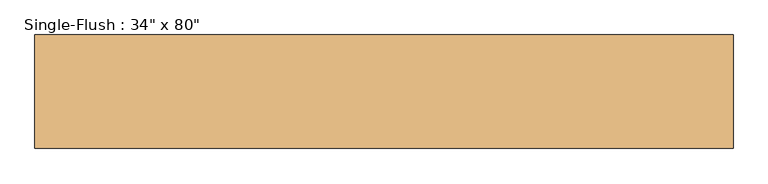
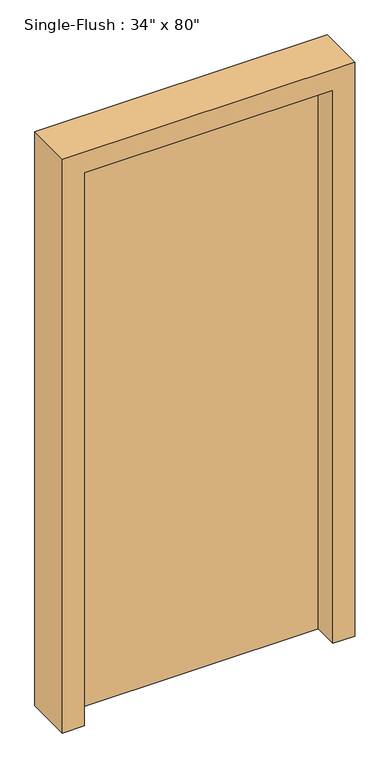
"""IFC4 building model written with IfcOpenShell, lengths in millimetres: door geometry."""

from ifc_helpers import new_model, si_unit, frame, origin, origin_with_axes, place, context, project, spatial, polyline, outline, extrude, source, transform, mapped, element, save


def door_d19e2db2(model_context):
    return source(origin(), model_context, "Body", "SweptSolid", [
        extrude(outline(polyline([(2108.2, 508.0), (2108.2, -508.0), (0.0, -508.0), (0.0, -431.8), (2032.0, -431.8), (2032.0, 431.8), (0.0, 431.8), (0.0, 508.0), (2108.2, 508.0)])), frame((0.0, -82.55, 0.0), z_axis=(0.0, 1.0, 0.0), x_axis=(0.0, 0.0, 1.0)), (0.0, 0.0, 1.0), 165.1),
        extrude(outline(polyline([(431.8, 6.35), (-431.8, 6.35), (-431.8, 57.15), (431.8, 57.15), (431.8, 6.35)])), origin_with_axes(), (0.0, 0.0, 1.0), 2032.0),
    ])


if __name__ == "__main__":
    model = new_model("IFC4")
    model_context = context("Model", 3, world=origin())
    ifc_project = project(units=[si_unit("LENGTHUNIT", "METRE", prefix="MILLI")], contexts=[model_context])
    site = spatial("IfcSite", under=ifc_project)
    building = spatial("IfcBuilding", under=site)
    placement = place(None, origin())
    door_shape = door_d19e2db2(model_context)
    element("IfcDoor", 1, ObjectType="Single-Flush : 34\" x 80\"", at=placement, inside=building, context=model_context, shape_type="MappedRepresentation", body=[
        mapped(door_shape, transform((0.0, 0.0, 0.0), x_axis=(1.0, 0.0, 0.0), y_axis=(0.0, 1.0, 0.0), z_axis=(0.0, 0.0, 1.0))),
    ])
    save(model, "model.ifc")

# Revit data of these elements
# Type "Single-Flush : 34\" x 80\""
#   Type Mark = "7"
#   OD_DS_Door_Material = "T.B.D."
#   OD_DS_Door_Type = "SWING"
#   OD_DS_Lockset = "PRIVACY LOCK"
#   Assembly Code = "C1020"
#   Analytic Construction = "<None>"
#   Thickness = 0' - 2"
#   RO Offset = 0' - 0 1/4"
#   Height = 6' - 8"
#   Trim Projection Ext = 0' - 1"
#   Trim Projection Int = 0' - 1"
#   Trim Width = 0' - 3"
#   Width = 2' - 10"
#   Door Material = Closet_1
#   Frame Material = Closet_1
#   Function = (empty or 0)
#   Wall Closure = (empty or 0)
# Element 1 (IfcDoor, "Single-Flush : 34\" x 80\"")
#   Materials on its faces: "Closet_1"
# Materials
#   "Closet_1": class "Paint", colour RGB 200 194 183, transparency 0, Cost = 0
